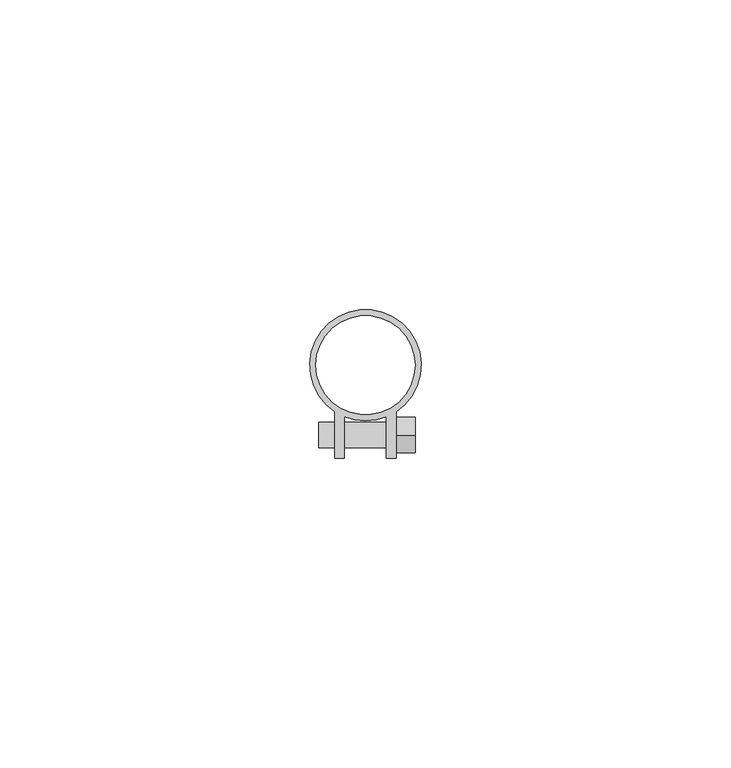
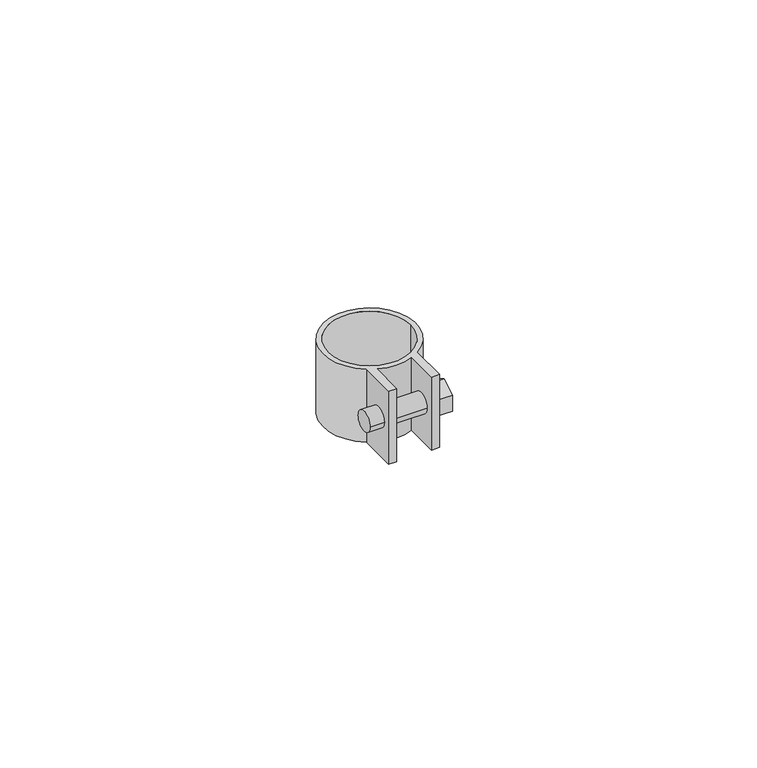
"""IFC4 building model written with IfcOpenShell, lengths in millimetres: proxy geometry, TN_Зажим для инъекционной трубки : TN_Зажим для инъекционной трубки."""

from ifc_helpers import new_model, si_unit, point, frame, frame_2d, origin, origin_with_axes, origin_2d, place, context, project, spatial, polyline, circle_curve, trimmed, segment, composite_curve, outline, extrude, source, transform, mapped, element, save


def specialty_equipment_d5bb3f4a(model_context):
    return source(origin(), model_context, "Body", "SweptSolid", [
        extrude(outline(polyline([(-8.4307015, 5.8587825), (-11.2733735, 4.2175651), (-14.1160456, 5.8587825), (-14.1160456, 9.1412175), (-11.2733735, 10.7824349), (-8.4307015, 9.1412175), (-8.4307015, 5.8587825)])), frame((4.9395193, 0.0, 0.0), z_axis=(1.0, 0.0, 0.0), x_axis=(0.0, 1.0, 0.0)), (0.0, 0.0, 1.0), 3.0604807),
        extrude(outline(composite_curve([segment(trimmed(circle_curve(frame_2d((-11.2733735, 7.5)), 2.0289427), [point((-13.3023162, 7.5))], [point((-9.2444309, 7.5))], False, "CARTESIAN"), True, "CONTINUOUS"), segment(trimmed(circle_curve(frame_2d((-11.2733735, 7.5)), 2.0289427), [point((-9.2444309, 7.5))], [point((-13.3023162, 7.5))], False, "CARTESIAN"), True, "CONTINUOUS")], self_intersect=False)), frame((-7.5205856, 0.0, 0.0), z_axis=(1.0, 0.0, 0.0), x_axis=(0.0, 1.0, 0.0)), (0.0, 0.0, 1.0), 12.4601049),
        extrude(outline(composite_curve([segment(trimmed(circle_curve(origin_2d(), 9.0), [point((3.3860062, -8.3387626))], [point((-3.3860062, -8.3387626))], False, "CARTESIAN"), True, "CONTINUOUS"), segment(polyline([(-3.3860062, -8.3387626), (-3.3860062, -15.0233735), (-4.9395193, -15.0233735), (-4.9395193, -7.5233735)]), True, "CONTINUOUS"), segment(trimmed(circle_curve(origin_2d(), 9.0), [point((-4.9395193, -7.5233735))], [point((4.9395193, -7.5233735))], False, "CARTESIAN"), True, "CONTINUOUS"), segment(polyline([(4.9395193, -7.5233735), (4.9395193, -15.0233735), (3.3860062, -15.0233735), (3.3860062, -8.3387626)]), True, "CONTINUOUS")], self_intersect=False), holes=[composite_curve([segment(trimmed(circle_curve(origin_2d(), 8.0), [point((-8.0, 0.0))], [point((8.0, 0.0))], True, "CARTESIAN"), True, "CONTINUOUS"), segment(trimmed(circle_curve(origin_2d(), 8.0), [point((8.0, 0.0))], [point((-8.0, 0.0))], True, "CARTESIAN"), True, "CONTINUOUS")], self_intersect=False)]), origin_with_axes(), (0.0, 0.0, 1.0), 15.0),
    ])


if __name__ == "__main__":
    model = new_model("IFC4")
    model_context = context("Model", 3, world=origin())
    ifc_project = project(units=[si_unit("LENGTHUNIT", "METRE", prefix="MILLI")], contexts=[model_context])
    site = spatial("IfcSite", under=ifc_project)
    building = spatial("IfcBuilding", under=site)
    placement = place(None, origin())
    specialty_equipment_shape = specialty_equipment_d5bb3f4a(model_context)
    element("IfcBuildingElementProxy", 1, Name="TN_Зажим для инъекционной трубки : TN_Зажим для инъекционной трубки", ObjectType="TN_Зажим для инъекционной трубки : TN_Зажим для инъекционной трубки", at=placement, inside=building, context=model_context, shape_type="MappedRepresentation", body=[
        mapped(specialty_equipment_shape, transform((0.0, 0.0, 0.0), x_axis=(1.0, 0.0, 0.0), y_axis=(0.0, 1.0, 0.0), z_axis=(0.0, 0.0, 1.0))),
    ])
    save(model, "model.ifc")

# Revit data of these elements
# Type "TN_Зажим для инъекционной трубки : TN_Зажим для инъекционной трубки"
#   Description = "Зажим для инъекционной трубки 10 мм"
#   Manufacturer = "ТехноНИКОЛЬ"
#   ADSK_Обозначение = "ТехноНИКОЛЬ"
#   ADSK_Наименование = "Зажим для инъекционной трубки 10 мм"
#   ADSK_Код изделия = ""
#   ADSK_Завод-изготовитель = "ТехноНИКОЛЬ"
#   ADSK_Единица измерения = "шт."
#   ADSK_Группирование = "Штуцеры и аксессуары"
#   ADSK_URL страницы изделия = ""
#   ADSK_URL документации изделия = ""
#   ADSK_Количество = 1
#   Материал = TN_СтальГальванизированная_Серый
#   Default Elevation = 0
#   URL = ""
# Element 1 (IfcBuildingElementProxy, "TN_Зажим для инъекционной трубки : TN_Зажим для инъекционной трубки")
#   Materials on its faces: "TN_СтальГальванизированная_Серый"
# Materials
#   "TN_СтальГальванизированная_Серый": class "Типовые", colour RGB 206 210 213, transparency 0, Cost = 0
